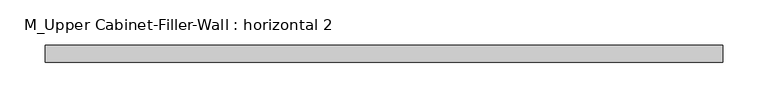
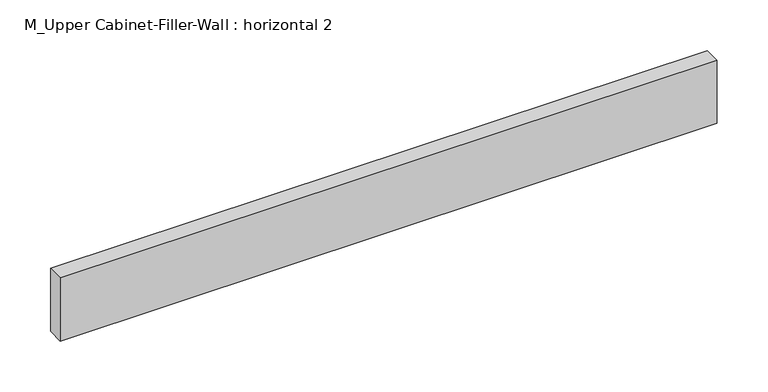
"""IFC4 building model written with IfcOpenShell, lengths in millimetres: furniture geometry, M_Upper Cabinet-Filler-Wall : horizontal 2."""

from ifc_helpers import new_model, si_unit, frame, origin, place, context, project, spatial, polyline, outline, extrude, source, transform, mapped, element, save


def m_upper_cabinet_filler_wall_horizontal_2_28a204f3(model_context):
    return source(origin(), model_context, "Body", "SweptSolid", [
        extrude(outline(polyline([(-344.8788372, 38.1), (-344.8788372, 57.15), (404.4211628, 57.15), (404.4211628, 38.1), (-344.8788372, 38.1)])), frame((0.0, 0.0, 1923.8), z_axis=(0.0, 0.0, 1.0), x_axis=(1.0, 0.0, 0.0)), (0.0, 0.0, 1.0), 76.2),
    ])


if __name__ == "__main__":
    model = new_model("IFC4")
    model_context = context("Model", 3, world=origin())
    ifc_project = project(units=[si_unit("LENGTHUNIT", "METRE", prefix="MILLI")], contexts=[model_context])
    site = spatial("IfcSite", under=ifc_project)
    building = spatial("IfcBuilding", under=site)
    placement = place(None, origin())
    m_upper_cabinet_filler_wall_horizontal_2_shape = m_upper_cabinet_filler_wall_horizontal_2_28a204f3(model_context)
    element("IfcFurniture", 1, ObjectType="M_Upper Cabinet-Filler-Wall : horizontal 2", at=placement, inside=building, context=model_context, shape_type="MappedRepresentation", body=[
        mapped(m_upper_cabinet_filler_wall_horizontal_2_shape, transform((0.0, 0.0, 0.0), x_axis=(1.0, 0.0, 0.0), y_axis=(0.0, 1.0, 0.0), z_axis=(0.0, 0.0, 1.0))),
    ])
    save(model, "model.ifc")

# Revit data of these elements
# Type "M_Upper Cabinet-Filler-Wall : horizontal 2"
#   Depth = 0' - 1"
#   Height = 0' - 3"
#   Top Of Cabinet = 6' - 6.74016"
#   Width = 2' - 5 1/2"
#   Cabinet Material = none
#   Default Elevation = 0
# Element 1 (IfcFurniture, "M_Upper Cabinet-Filler-Wall : horizontal 2")
#   Materials on its faces: "Cabinets"
# Materials
#   "Cabinets": class "Miscellaneous", colour RGB 249 249 249, transparency 0
